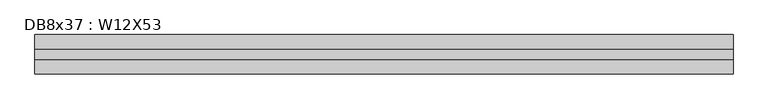
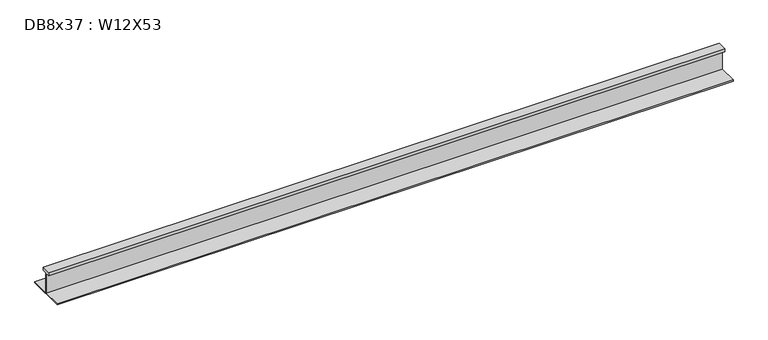
"""IFC4 building model written with IfcOpenShell, lengths in millimetres: beam geometry, DB8x37 : W12X53."""

from ifc_helpers import new_model, si_unit, frame, origin, place, context, project, spatial, polyline, outline, extrude, source, transform, mapped, element, save


def db8x37_w12x53_03f9f2bd(model_context):
    return source(origin(), model_context, "Body", "SweptSolid", [
        extrude(outline(polyline([(38.1, 145.415), (38.1, 120.015), (2.921, 120.015), (2.921, -48.4505), (152.4, -48.4505), (152.4, -58.1025), (-152.4, -58.1025), (-152.4, -48.4505), (-2.921, -48.4505), (-2.921, 120.015), (-38.1, 120.015), (-38.1, 145.415), (38.1, 145.415)])), frame((-2703.83, 0.0, 0.0), z_axis=(1.0, 0.0, 0.0), x_axis=(0.0, 1.0, 0.0)), (0.0, 0.0, 1.0), 5382.26),
    ])


if __name__ == "__main__":
    model = new_model("IFC4")
    model_context = context("Model", 3, world=origin())
    ifc_project = project(units=[si_unit("LENGTHUNIT", "METRE", prefix="MILLI")], contexts=[model_context])
    site = spatial("IfcSite", under=ifc_project)
    building = spatial("IfcBuilding", under=site)
    placement = place(None, origin())
    db8x37_w12x53_shape = db8x37_w12x53_03f9f2bd(model_context)
    element("IfcBeam", 1, ObjectType="DB8x37 : W12X53", at=placement, inside=building, context=model_context, shape_type="MappedRepresentation", body=[
        mapped(db8x37_w12x53_shape, transform((0.0, 0.0, 0.0), x_axis=(1.0, 0.0, 0.0), y_axis=(0.0, 1.0, 0.0), z_axis=(0.0, 0.0, 1.0))),
    ])
    save(model, "model.ifc")

# Revit data of these elements
# Type "DB8x37 : W12X53"
#   Assembly Code = "B10"
#   W = 53
#   Length [instance default] = 5' - 0"
#   bf = 0' - 10"
#   d = 1' - 0.1"
#   k = 0' - 1 3/8"
#   k2 = 0' - 0.8"
#   tf = 0' - 0.575"
#   tw = 0' - 0.345"
#   A = 0.108333 SF
#   Structural Material [instance default] = Steel ASTM A992
# Element 1 (IfcBeam, "DB8x37 : W12X53")
#   Materials on its faces: "Steel ASTM A992"
# Materials
#   "Steel ASTM A992": class "Metal", colour RGB 199 199 199, transparency 0, Description = "Structural steel 50ksi", Cost = 0
